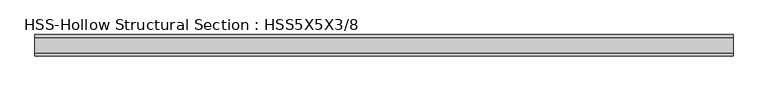
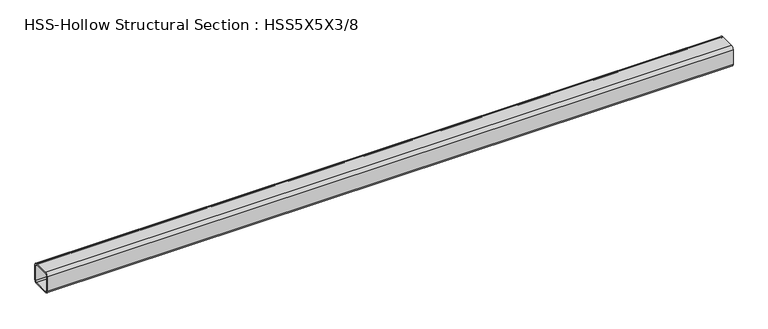
"""IFC4 building model written with IfcOpenShell, lengths in millimetres: member geometry, HSS-Hollow Structural Section : HSS5X5X3/8."""

from ifc_helpers import new_model, si_unit, point, frame, frame_2d, origin, place, context, project, spatial, polyline, circle_curve, trimmed, segment, composite_curve, outline, extrude, source, transform, mapped, element, save


def hss_hollow_structural_section_hss5x5x3_8_ba72fdac(model_context):
    return source(origin(), model_context, "Body", "SweptSolid", [
        extrude(outline(composite_curve([segment(polyline([(63.5, 45.7708), (63.5, -45.7708)]), True, "CONTINUOUS"), segment(trimmed(circle_curve(frame_2d((45.7708, -45.7708)), 17.7292), [point((63.5, -45.7708))], [point((45.7708, -63.5))], False, "CARTESIAN"), True, "CONTINUOUS"), segment(polyline([(45.7708, -63.5), (-45.7708, -63.5)]), True, "CONTINUOUS"), segment(trimmed(circle_curve(frame_2d((-45.7708, -45.7708)), 17.7292), [point((-45.7708, -63.5))], [point((-63.5, -45.7708))], False, "CARTESIAN"), True, "CONTINUOUS"), segment(polyline([(-63.5, -45.7708), (-63.5, 45.7708)]), True, "CONTINUOUS"), segment(trimmed(circle_curve(frame_2d((-45.7708, 45.7708)), 17.7292), [point((-63.5, 45.7708))], [point((-45.7708, 63.5))], False, "CARTESIAN"), True, "CONTINUOUS"), segment(polyline([(-45.7708, 63.5), (45.7708, 63.5)]), True, "CONTINUOUS"), segment(trimmed(circle_curve(frame_2d((45.7708, 45.7708)), 17.7292), [point((45.7708, 63.5))], [point((63.5, 45.7708))], False, "CARTESIAN"), True, "CONTINUOUS")], self_intersect=False), holes=[composite_curve([segment(trimmed(circle_curve(frame_2d((-45.7708, 45.7708)), 8.8646), [point((-45.7708, 54.6354))], [point((-54.6354, 45.7708))], True, "CARTESIAN"), True, "CONTINUOUS"), segment(polyline([(-54.6354, 45.7708), (-54.6354, -45.7708)]), True, "CONTINUOUS"), segment(trimmed(circle_curve(frame_2d((-45.7708, -45.7708)), 8.8646), [point((-54.6354, -45.7708))], [point((-45.7708, -54.6354))], True, "CARTESIAN"), True, "CONTINUOUS"), segment(polyline([(-45.7708, -54.6354), (45.7708, -54.6354)]), True, "CONTINUOUS"), segment(trimmed(circle_curve(frame_2d((45.7708, -45.7708)), 8.8646), [point((45.7708, -54.6354))], [point((54.6354, -45.7708))], True, "CARTESIAN"), True, "CONTINUOUS"), segment(polyline([(54.6354, -45.7708), (54.6354, 45.7708)]), True, "CONTINUOUS"), segment(trimmed(circle_curve(frame_2d((45.7708, 45.7708)), 8.8646), [point((54.6354, 45.7708))], [point((45.7708, 54.6354))], True, "CARTESIAN"), True, "CONTINUOUS"), segment(polyline([(45.7708, 54.6354), (-45.7708, 54.6354)]), True, "CONTINUOUS")], self_intersect=False)]), frame((-2069.3907215, 0.0, 0.0), z_axis=(1.0, 0.0, 0.0), x_axis=(0.0, 1.0, 0.0)), (0.0, 0.0, 1.0), 4138.7814431),
    ])


if __name__ == "__main__":
    model = new_model("IFC4")
    model_context = context("Model", 3, world=origin())
    ifc_project = project(units=[si_unit("LENGTHUNIT", "METRE", prefix="MILLI")], contexts=[model_context])
    site = spatial("IfcSite", under=ifc_project)
    building = spatial("IfcBuilding", under=site)
    placement = place(None, origin())
    hss_hollow_structural_section_hss5x5x3_8_shape = hss_hollow_structural_section_hss5x5x3_8_ba72fdac(model_context)
    element("IfcMember", 1, ObjectType="HSS-Hollow Structural Section : HSS5X5X3/8", at=placement, inside=building, context=model_context, shape_type="MappedRepresentation", body=[
        mapped(hss_hollow_structural_section_hss5x5x3_8_shape, transform((0.0, 0.0, 0.0), x_axis=(1.0, 0.0, 0.0), y_axis=(0.0, 1.0, 0.0), z_axis=(0.0, 0.0, 1.0))),
    ])
    save(model, "model.ifc")

# Revit data of these elements
# Type "HSS-Hollow Structural Section : HSS5X5X3/8"
#   Assembly Code = "B10"
#   Shape = "Square"
#   W = 22.3
#   Ht = 0' - 5"
#   Length [instance default] = 5' - 0"
#   b = 0' - 5"
#   kr = 0' - 0.698"
#   t = 0' - 0.349"
#   A = 0.0429167 SF
#   Structural Material [instance default] = Steel ASTM A500, Grade B, Rectangular and Square
# Element 1 (IfcMember, "HSS-Hollow Structural Section : HSS5X5X3/8")
#   Materials on its faces: "Steel ASTM A500, Grade B, Rectangular and Square"
# Materials
#   "Steel ASTM A500, Grade B, Rectangular and Square": class "Metal", colour RGB 199 199 199, transparency 0, Description = "Carbon steel", Cost = 0
